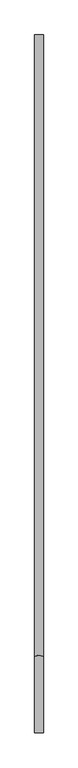
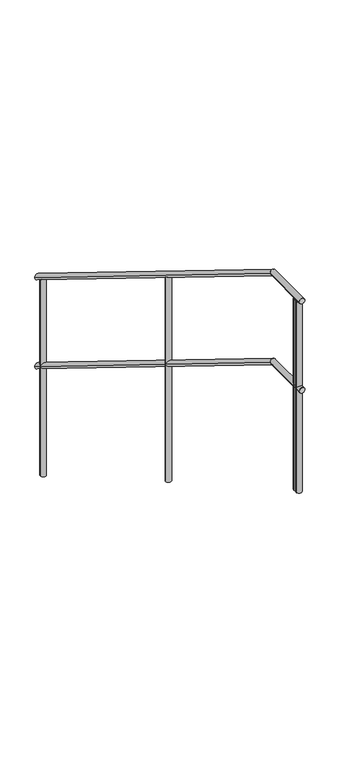
"""IFC4 building model written with IfcOpenShell, lengths in millimetres: railing geometry."""

from ifc_helpers import new_model, si_unit, point, frame, frame_2d, origin, place, context, project, spatial, circle_curve, ellipse_curve, trimmed, segment, composite_curve, outline, extrude, source, transform, mapped, element, save
from ifc_brep_helpers import plane_surface, cylinder_surface, advanced_brep


def railing_c8857c04(model_context):
    return source(origin(), model_context, "Body", "SolidModel", [
        advanced_brep(
        [(-1026.0, 15342.7934796, -450.9609787), (-1056.0, 15342.7934796, -450.9609787), (-1056.0, 13178.5366941, 885.0), (-1026.0, 13178.5366941, 885.0), (-1026.0, 12912.7934796, 885.0), (-1056.0, 12912.7934796, 885.0)],
        [
            (0, 1, ellipse_curve(frame((-1041.0, 15342.7934796, -450.9609787), z_axis=(0.0, 1.0, 0.0), x_axis=(0.0, 0.0, -1.0)), 17.6276454, 15.0)),
            (1, 0, ellipse_curve(frame((-1041.0, 15342.7934796, -450.9609787), z_axis=(0.0, 1.0, 0.0), x_axis=(0.0, 0.0, -1.0)), 17.6276454, 15.0)),
            (1, 2),
            (2, 3, ellipse_curve(frame((-1041.0, 13178.5366941, 885.0), z_axis=(0.0, 0.9620125025549408, -0.2730053935877093), x_axis=(0.0, -0.27300539358770903, -0.962012502554941)), 15.5923129, 15.0)),
            (3, 0),
            (3, 2, ellipse_curve(frame((-1041.0, 13178.5366941, 885.0), z_axis=(0.0, 0.9620125025549408, -0.2730053935877093), x_axis=(0.0, -0.27300539358770903, -0.962012502554941)), 15.5923129, 15.0)),
            (4, 5, circle_curve(frame((-1041.0, 12912.7934796, 885.0), z_axis=(0.0, -1.0, 0.0), x_axis=(-1.0, 0.0, 0.0)), 15.0)),
            (5, 4, circle_curve(frame((-1041.0, 12912.7934796, 885.0), z_axis=(0.0, -1.0, 0.0), x_axis=(-1.0, 0.0, 0.0)), 15.0)),
            (2, 5),
            (4, 3),
        ],
        [
            plane_surface(frame((-1041.0, 15342.7934796, -433.3333333), z_axis=(0.0, 1.0, 0.0), x_axis=(0.0, 0.0, -1.0))),
            cylinder_surface(frame((-1041.0, 15334.9144415, -446.097375), z_axis=(0.0, 0.8509361101440399, -0.5252692037926177), x_axis=(-1.0, 0.0, 0.0)), 15.0),
            plane_surface(frame((-1041.0, 12912.7934796, 900.0), z_axis=(0.0, -1.0, 0.0), x_axis=(0.0, 0.0, -1.0))),
            cylinder_surface(frame((-1041.0, 13182.7934796, 885.0), z_axis=(0.0, 1.0, 0.0), x_axis=(-1.0, 0.0, 0.0)), 15.0),
        ],
        [
            (0, [[1, 2]]),
            (1, [[-2, 3, 4, 5]]),
            (1, [[-1, -5, 6, -3]]),
            (2, [[7, 8]]),
            (3, [[-4, 9, -7, 10]]),
            (3, [[-6, -10, -8, -9]]),
        ],
    ),
        advanced_brep(
        [(-1026.0, 15342.7934796, 49.0390213), (-1056.0, 15342.7934796, 49.0390213), (-1056.0, 13178.5366941, 1385.0), (-1026.0, 13178.5366941, 1385.0), (-1026.0, 12912.7934796, 1385.0), (-1056.0, 12912.7934796, 1385.0)],
        [
            (0, 1, ellipse_curve(frame((-1041.0, 15342.7934796, 49.0390213), z_axis=(0.0, 1.0, 0.0), x_axis=(0.0, 0.0, -1.0)), 17.6276454, 15.0)),
            (1, 0, ellipse_curve(frame((-1041.0, 15342.7934796, 49.0390213), z_axis=(0.0, 1.0, 0.0), x_axis=(0.0, 0.0, -1.0)), 17.6276454, 15.0)),
            (1, 2),
            (2, 3, ellipse_curve(frame((-1041.0, 13178.5366941, 1385.0), z_axis=(0.0, 0.9620125025549408, -0.2730053935877093), x_axis=(0.0, -0.27300539358770903, -0.962012502554941)), 15.5923129, 15.0)),
            (3, 0),
            (3, 2, ellipse_curve(frame((-1041.0, 13178.5366941, 1385.0), z_axis=(0.0, 0.9620125025549408, -0.2730053935877093), x_axis=(0.0, -0.27300539358770903, -0.962012502554941)), 15.5923129, 15.0)),
            (4, 5, circle_curve(frame((-1041.0, 12912.7934796, 1385.0), z_axis=(0.0, -1.0, 0.0), x_axis=(-1.0, 0.0, 0.0)), 15.0)),
            (5, 4, circle_curve(frame((-1041.0, 12912.7934796, 1385.0), z_axis=(0.0, -1.0, 0.0), x_axis=(-1.0, 0.0, 0.0)), 15.0)),
            (2, 5),
            (4, 3),
        ],
        [
            plane_surface(frame((-1041.0, 15342.7934796, 66.6666667), z_axis=(0.0, 1.0, 0.0), x_axis=(0.0, 0.0, -1.0))),
            cylinder_surface(frame((-1041.0, 15334.9144415, 53.902625), z_axis=(0.0, 0.8509361101440399, -0.5252692037926177), x_axis=(-1.0, 0.0, 0.0)), 15.0),
            plane_surface(frame((-1041.0, 12912.7934796, 1400.0), z_axis=(0.0, -1.0, 0.0), x_axis=(0.0, 0.0, -1.0))),
            cylinder_surface(frame((-1041.0, 13182.7934796, 1385.0), z_axis=(0.0, 1.0, 0.0), x_axis=(-1.0, 0.0, 0.0)), 15.0),
        ],
        [
            (0, [[1, 2]]),
            (1, [[-2, 3, 4, 5]]),
            (1, [[-1, -5, 6, -3]]),
            (2, [[7, 8]]),
            (3, [[-4, 9, -7, 10]]),
            (3, [[-6, -10, -8, -9]]),
        ],
    ),
        extrude(outline(composite_curve([segment(trimmed(circle_curve(frame_2d((-1041.0, 12942.7934796)), 15.0), [point((-1026.0, 12942.7934796))], [point((-1056.0, 12942.7934796))], False, "CARTESIAN"), True, "CONTINUOUS"), segment(trimmed(circle_curve(frame_2d((-1041.0, 12942.7934796)), 15.0), [point((-1056.0, 12942.7934796))], [point((-1026.0, 12942.7934796))], False, "CARTESIAN"), True, "CONTINUOUS")], self_intersect=False)), frame((0.0, 0.0, 300.0), z_axis=(0.0, 0.0, 1.0), x_axis=(1.0, 0.0, 0.0)), (0.0, 0.0, 1.0), 1070.0),
        advanced_brep(
        [(-1056.0, 14142.7934796, 777.4074074), (-1056.0, 14142.7934796, -366.6666667), (-1026.0, 14142.7934796, -366.6666667), (-1026.0, 14142.7934796, 777.4074074)],
        [
            (0, 1),
            (1, 2, circle_curve(frame((-1041.0, 14142.7934796, -366.6666667), z_axis=(0.0, 0.0, 1.0), x_axis=(1.0, 0.0, 0.0)), 15.0)),
            (2, 3),
            (3, 0, ellipse_curve(frame((-1041.0, 14142.7934796, 777.4074074), z_axis=(0.0, -0.5252692037926167, -0.8509361101440406), x_axis=(0.0, -0.8509361101440406, 0.5252692037926162)), 17.6276454, 15.0)),
            (0, 3, ellipse_curve(frame((-1041.0, 14142.7934796, 777.4074074), z_axis=(0.0, -0.5252692037926167, -0.8509361101440406), x_axis=(0.0, -0.8509361101440406, 0.5252692037926162)), 17.6276454, 15.0)),
            (2, 1, circle_curve(frame((-1041.0, 14142.7934796, -366.6666667), z_axis=(0.0, 0.0, 1.0), x_axis=(1.0, 0.0, 0.0)), 15.0)),
        ],
        [
            cylinder_surface(frame((-1041.0, 14142.7934796, -466.6666667), z_axis=(0.0, 0.0, 1.0), x_axis=(1.0, 0.0, 0.0)), 15.0),
            plane_surface(frame((-1016.0, 14117.7934796, 792.8395062), z_axis=(0.0, 0.5252692037926167, 0.8509361101440406), x_axis=(-1.0, 0.0, 0.0))),
            plane_surface(frame((-1016.0, 14167.7934796, -366.6666667), z_axis=(0.0, 0.0, -1.0), x_axis=(-1.0, 0.0, 0.0))),
        ],
        [
            (0, [[1, 2, 3, 4]]),
            (0, [[-1, 5, -3, 6]]),
            (1, [[-4, -5]]),
            (2, [[-2, -6]]),
        ],
    ),
        extrude(outline(composite_curve([segment(trimmed(circle_curve(frame_2d((-1041.0, 12962.7934796)), 15.0), [point((-1026.0, 12962.7934796))], [point((-1056.0, 12962.7934796))], False, "CARTESIAN"), True, "CONTINUOUS"), segment(trimmed(circle_curve(frame_2d((-1041.0, 12962.7934796)), 15.0), [point((-1056.0, 12962.7934796))], [point((-1026.0, 12962.7934796))], False, "CARTESIAN"), True, "CONTINUOUS")], self_intersect=False)), frame((0.0, 0.0, 300.0), z_axis=(0.0, 0.0, 1.0), x_axis=(1.0, 0.0, 0.0)), (0.0, 0.0, 1.0), 1070.0),
        advanced_brep(
        [(-1056.0, 15292.7934796, 67.5308642), (-1056.0, 15292.7934796, -1033.3333333), (-1026.0, 15292.7934796, -1033.3333333), (-1026.0, 15292.7934796, 67.5308642)],
        [
            (0, 1),
            (1, 2, circle_curve(frame((-1041.0, 15292.7934796, -1033.3333333), z_axis=(0.0, 0.0, 1.0), x_axis=(1.0, 0.0, 0.0)), 15.0)),
            (2, 3),
            (3, 0, ellipse_curve(frame((-1041.0, 15292.7934796, 67.5308642), z_axis=(0.0, -0.5252692037926167, -0.8509361101440406), x_axis=(0.0, -0.8509361101440406, 0.5252692037926162)), 17.6276454, 15.0)),
            (0, 3, ellipse_curve(frame((-1041.0, 15292.7934796, 67.5308642), z_axis=(0.0, -0.5252692037926167, -0.8509361101440406), x_axis=(0.0, -0.8509361101440406, 0.5252692037926162)), 17.6276454, 15.0)),
            (2, 1, circle_curve(frame((-1041.0, 15292.7934796, -1033.3333333), z_axis=(0.0, 0.0, 1.0), x_axis=(1.0, 0.0, 0.0)), 15.0)),
        ],
        [
            cylinder_surface(frame((-1041.0, 15292.7934796, -1133.3333333), z_axis=(0.0, 0.0, 1.0), x_axis=(1.0, 0.0, 0.0)), 15.0),
            plane_surface(frame((-1016.0, 15267.7934796, 82.962963), z_axis=(0.0, 0.5252692037926167, 0.8509361101440406), x_axis=(-1.0, 0.0, 0.0))),
            plane_surface(frame((-1016.0, 15317.7934796, -1033.3333333), z_axis=(0.0, 0.0, -1.0), x_axis=(-1.0, 0.0, 0.0))),
        ],
        [
            (0, [[1, 2, 3, 4]]),
            (0, [[-1, 5, -3, 6]]),
            (1, [[-4, -5]]),
            (2, [[-2, -6]]),
        ],
    ),
    ])


if __name__ == "__main__":
    model = new_model("IFC4")
    model_context = context("Model", 3, world=origin())
    ifc_project = project(units=[si_unit("LENGTHUNIT", "METRE", prefix="MILLI")], contexts=[model_context])
    site = spatial("IfcSite", under=ifc_project)
    building = spatial("IfcBuilding", under=site)
    placement = place(None, origin())
    railing_shape = railing_c8857c04(model_context)
    element("IfcRailing", 1, at=placement, inside=building, context=model_context, shape_type="MappedRepresentation", body=[
        mapped(railing_shape, transform((0.0, 0.0, 0.0), x_axis=(1.0, 0.0, 0.0), y_axis=(0.0, 1.0, 0.0), z_axis=(0.0, 0.0, 1.0))),
    ])
    save(model, "model.ifc")
